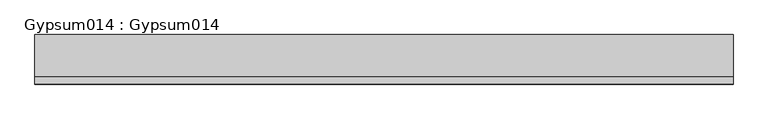
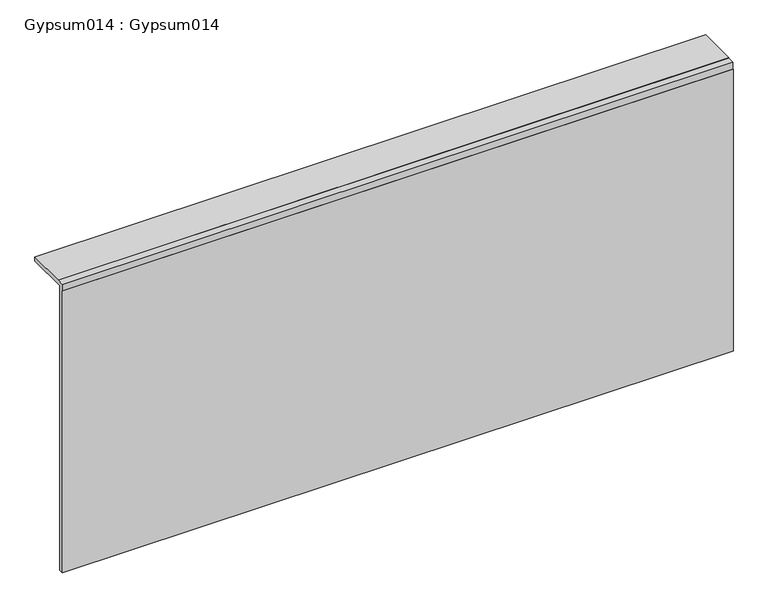
"""IFC4 building model written with IfcOpenShell, lengths in millimetres: proxy geometry, Gypsum014 : Gypsum014."""

from ifc_helpers import new_model, si_unit, frame, origin, place, context, project, spatial, polyline, outline, extrude, source, transform, mapped, element, save


def gypsum014_gypsum014_2fa6baae(model_context):
    return source(origin(), model_context, "Body", "SweptSolid", [
        extrude(outline(polyline([(9576.3500834, 36602.466), (9576.3500834, 37490.9066598), (9577.6300834, 37490.9066598), (9577.6300834, 37512.0598438), (9598.7832673, 37512.0598438), (9598.7832673, 37513.3398438), (9718.4918386, 37513.3398438), (9718.4918386, 37500.1015625), (9590.6383229, 37500.1015625), (9590.6383229, 36602.466), (9576.3500834, 36602.466)])), frame((3694.2883192, 0.0, 0.0), z_axis=(1.0, 0.0, 0.0), x_axis=(0.0, 1.0, 0.0)), (0.0, 0.0, 1.0), 2000.0),
    ])


if __name__ == "__main__":
    model = new_model("IFC4")
    model_context = context("Model", 3, world=origin())
    ifc_project = project(units=[si_unit("LENGTHUNIT", "METRE", prefix="MILLI")], contexts=[model_context])
    site = spatial("IfcSite", under=ifc_project)
    building = spatial("IfcBuilding", under=site)
    placement = place(None, origin())
    gypsum014_gypsum014_shape = gypsum014_gypsum014_2fa6baae(model_context)
    element("IfcBuildingElementProxy", 1, Name="Gypsum014 : Gypsum014", ObjectType="Gypsum014 : Gypsum014", at=placement, inside=building, context=model_context, shape_type="MappedRepresentation", body=[
        mapped(gypsum014_gypsum014_shape, transform((0.0, 0.0, 0.0), x_axis=(1.0, 0.0, 0.0), y_axis=(0.0, 1.0, 0.0), z_axis=(0.0, 0.0, 1.0))),
    ])
    save(model, "model.ifc")

# Revit data of these elements
# Type "Gypsum014 : Gypsum014"
#   NameOverride = "Gypsum014"
# Element 1 (IfcBuildingElementProxy, "Gypsum014 : Gypsum014")
#   Materials on its faces: "5/8\" GYPSUM BOARD"
# Materials
#   "5/8\" GYPSUM BOARD": class "Unassigned", colour RGB 214 214 214, transparency 0, Cost = 0
